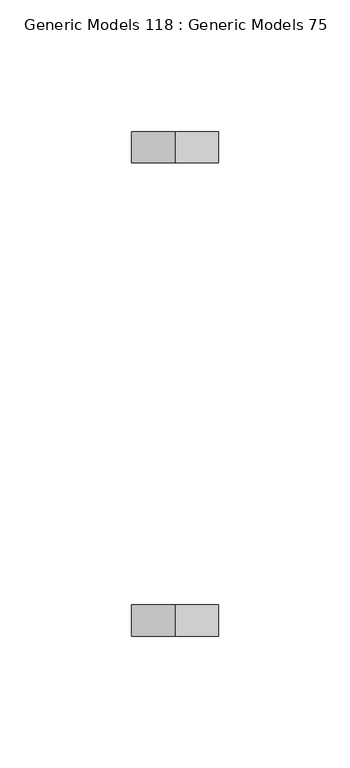
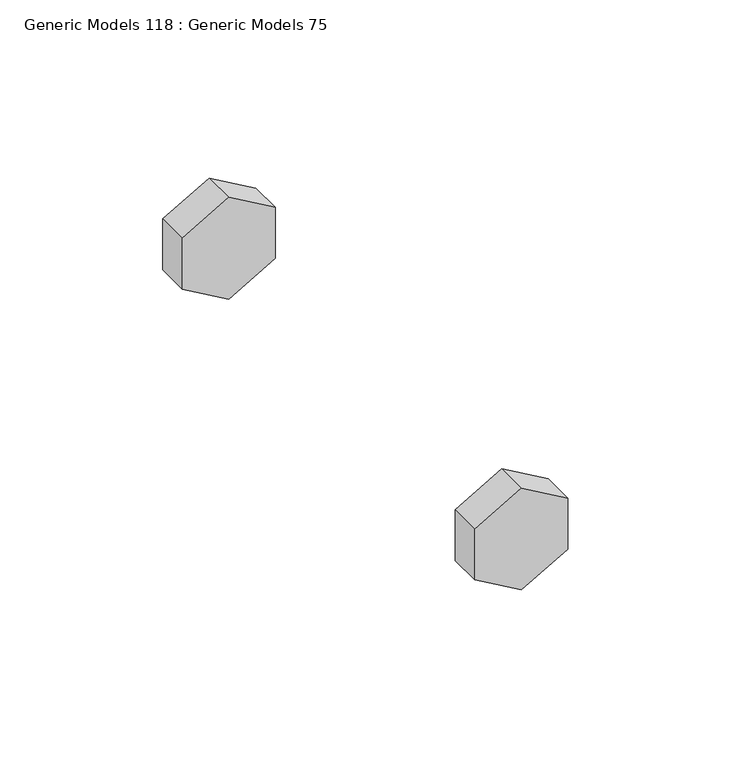
"""IFC4 building model written with IfcOpenShell, lengths in millimetres: proxy geometry, Generic Models 118 : Generic Models 75."""

from ifc_helpers import new_model, si_unit, frame, origin, place, context, project, spatial, polyline, outline, extrude, source, transform, mapped, element, save


def generic_models_118_generic_models_75_bcc7ce39(model_context):
    return source(origin(), model_context, "Body", "SweptSolid", [
        extrude(outline(polyline([(269389.225, 31991.9073871), (269408.275, 31991.9073871), (269417.8, 31975.4096032), (269408.275, 31958.9118192), (269389.225, 31958.9118192), (269379.7, 31975.4096032), (269389.225, 31991.9073871)])), frame((0.0, 30858.4781612, 0.0), z_axis=(0.0, 1.0, 0.0), x_axis=(0.0, 0.0, 1.0)), (0.0, 0.0, 1.0), 11.90625),
        extrude(outline(polyline([(269389.225, 31991.9073871), (269408.275, 31991.9073871), (269417.8, 31975.4096032), (269408.275, 31958.9118192), (269389.225, 31958.9118192), (269379.7, 31975.4096032), (269389.225, 31991.9073871)])), frame((0.0, 30678.6937862, 0.0), z_axis=(0.0, 1.0, 0.0), x_axis=(0.0, 0.0, 1.0)), (0.0, 0.0, 1.0), 11.90625),
    ])


if __name__ == "__main__":
    model = new_model("IFC4")
    model_context = context("Model", 3, world=origin())
    ifc_project = project(units=[si_unit("LENGTHUNIT", "METRE", prefix="MILLI")], contexts=[model_context])
    site = spatial("IfcSite", under=ifc_project)
    building = spatial("IfcBuilding", under=site)
    placement = place(None, origin())
    generic_models_118_generic_models_75_shape = generic_models_118_generic_models_75_bcc7ce39(model_context)
    element("IfcBuildingElementProxy", 1, Name="Generic Models 118 : Generic Models 75", ObjectType="Generic Models 118 : Generic Models 75", at=placement, inside=building, context=model_context, shape_type="MappedRepresentation", body=[
        mapped(generic_models_118_generic_models_75_shape, transform((0.0, 0.0, 0.0), x_axis=(1.0, 0.0, 0.0), y_axis=(0.0, 1.0, 0.0), z_axis=(0.0, 0.0, 1.0))),
    ])
    save(model, "model.ifc")
